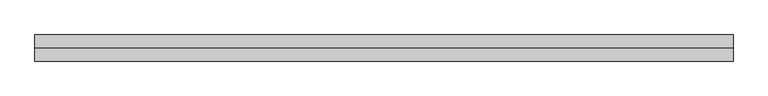
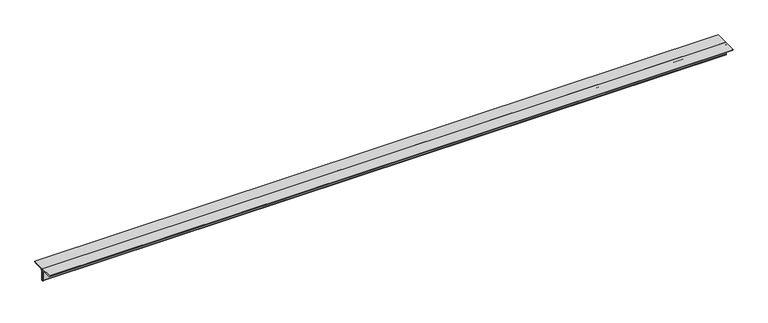
"""IFC4 building model written with IfcOpenShell, lengths in millimetres: member geometry, Steel Framing_2Ls_KS : H_SB_AR_S02_2Ls-100x100x10_VBR1."""

from ifc_helpers import new_model, si_unit, point, frame, frame_2d, origin, place, context, project, spatial, polyline, circle_curve, trimmed, segment, composite_curve, outline, extrude, source, transform, mapped, element, save


def member_09b5a921(model_context):
    return source(origin(), model_context, "Body", "SweptSolid", [
        extrude(outline(composite_curve([segment(polyline([(0.0, 28.2), (100.0, 28.2)]), True, "CONTINUOUS"), segment(trimmed(circle_curve(frame_2d((90.0, 28.2)), 10.0), [point((100.0, 28.2))], [point((90.0, 18.2))], False, "CARTESIAN"), True, "CONTINUOUS"), segment(polyline([(90.0, 18.2), (20.0, 18.2)]), True, "CONTINUOUS"), segment(trimmed(circle_curve(frame_2d((20.0, 8.2)), 10.0), [point((20.0, 18.2))], [point((10.0, 8.2))], True, "CARTESIAN"), True, "CONTINUOUS"), segment(polyline([(10.0, 8.2), (10.0, -61.8)]), True, "CONTINUOUS"), segment(trimmed(circle_curve(frame_2d((0.0, -61.8)), 10.0), [point((10.0, -61.8))], [point((0.0, -71.8))], False, "CARTESIAN"), True, "CONTINUOUS"), segment(polyline([(0.0, -71.8), (0.0, 28.2)]), True, "CONTINUOUS")], self_intersect=False)), frame((-2590.3354834, 0.0, 0.0), z_axis=(1.0, 0.0, 0.0), x_axis=(0.0, 1.0, 0.0)), (0.0, 0.0, 1.0), 5345.6471524),
        extrude(outline(composite_curve([segment(polyline([(0.0, 28.2), (0.0, -71.8)]), True, "CONTINUOUS"), segment(trimmed(circle_curve(frame_2d((0.0, -61.8)), 10.0), [point((0.0, -71.8))], [point((-10.0, -61.8))], False, "CARTESIAN"), True, "CONTINUOUS"), segment(polyline([(-10.0, -61.8), (-10.0, 8.2)]), True, "CONTINUOUS"), segment(trimmed(circle_curve(frame_2d((-20.0, 8.2)), 10.0), [point((-10.0, 8.2))], [point((-20.0, 18.2))], True, "CARTESIAN"), True, "CONTINUOUS"), segment(polyline([(-20.0, 18.2), (-90.0, 18.2)]), True, "CONTINUOUS"), segment(trimmed(circle_curve(frame_2d((-90.0, 28.2)), 10.0), [point((-90.0, 18.2))], [point((-100.0, 28.2))], False, "CARTESIAN"), True, "CONTINUOUS"), segment(polyline([(-100.0, 28.2), (0.0, 28.2)]), True, "CONTINUOUS")], self_intersect=False)), frame((-2590.3354834, 0.0, 0.0), z_axis=(1.0, 0.0, 0.0), x_axis=(0.0, 1.0, 0.0)), (0.0, 0.0, 1.0), 5345.6471524),
    ])


if __name__ == "__main__":
    model = new_model("IFC4")
    model_context = context("Model", 3, world=origin())
    ifc_project = project(units=[si_unit("LENGTHUNIT", "METRE", prefix="MILLI")], contexts=[model_context])
    site = spatial("IfcSite", under=ifc_project)
    building = spatial("IfcBuilding", under=site)
    placement = place(None, origin())
    member_shape = member_09b5a921(model_context)
    element("IfcMember", 1, ObjectType="Steel Framing_2Ls_KS : H_SB_AR_S02_2Ls-100x100x10_VBR1", at=placement, inside=building, context=model_context, shape_type="MappedRepresentation", body=[
        mapped(member_shape, transform((0.0, 0.0, 0.0), x_axis=(1.0, 0.0, 0.0), y_axis=(0.0, 1.0, 0.0), z_axis=(0.0, 0.0, 1.0))),
    ])
    save(model, "model.ifc")

# Revit data of these elements
# Type "Steel Framing_2Ls_KS : H_SB_AR_S02_2Ls-100x100x10_VBR1"
#   Type Comments = "MAIN"
#   Type Mark = "VBR1"
#   H_SectionID = "2Ls-100x100x10"
#   Assembly Code = "B10"
#   Legs = "LLBB"
#   H_Ratio for Additional Steel Plate = 0.2
#   W = 0
#   Perimeter = 0.80 m²/m
#   Nominal Weight = 29.80 kgf/m
#   Length [instance default] = 1524 mm
#   Space = 0 mm
#   b = 100 mm
#   d = 100 mm
#   t = 10 mm
#   y = 28.2 mm
#   A = 0.0038 m²
#   Structural Material [instance default] = Steel, 45-345
# Element 1 (IfcMember, "Steel Framing_2Ls_KS : H_SB_AR_S02_2Ls-100x100x10_VBR1")
#   Materials on its faces: "Steel, 45-345"
# Materials
#   "Steel, 45-345": class "Metal", colour RGB 189 187 185, transparency 0, Description = "Steel 345 MPa", Cost = 0
